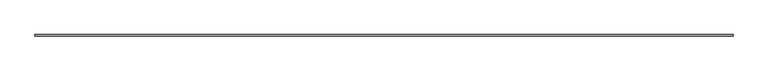
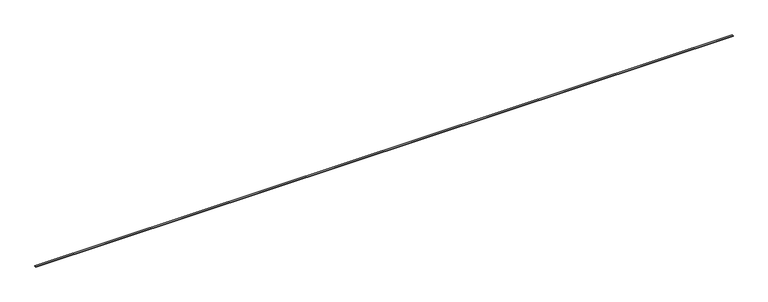
"""IFC4 building model written with IfcOpenShell, lengths in millimetres: proxy geometry, Generic Models 7:Generic Models 1:2:Generic Models 1:2 : Generic Models 7:Generic Models 1:337419:2 : Generic Models 7:Generic Models 1:2:Generic Models 1:2 : Generic Models 7:Generic Models 1:337419:306751."""

from ifc_helpers import new_model, si_unit, frame, origin, place, context, project, spatial, polyline, outline, extrude, source, transform, mapped, element, save


def generic_models_2ad7ca59(model_context):
    return source(origin(), model_context, "Body", "SweptSolid", [
        extrude(outline(polyline([(0.0, -164.8422109), (0.0, 0.0), (76200.0204281, 0.0), (76200.0204281, -164.8422109), (0.0, -164.8422109)])), frame((667506.057152, -567050.5861887, 8571.3891581), z_axis=(0.0, -0.041630544767773385, 0.9991330730900356), x_axis=(-1.0, 0.0, 0.0)), (0.0, 0.0, 1.0), 38.1),
    ])


if __name__ == "__main__":
    model = new_model("IFC4")
    model_context = context("Model", 3, world=origin())
    ifc_project = project(units=[si_unit("LENGTHUNIT", "METRE", prefix="MILLI")], contexts=[model_context])
    site = spatial("IfcSite", under=ifc_project)
    building = spatial("IfcBuilding", under=site)
    placement = place(None, origin())
    generic_models_shape = generic_models_2ad7ca59(model_context)
    element("IfcBuildingElementProxy", 1, Name="Generic Models 7:Generic Models 1:2:Generic Models 1:2 : Generic Models 7:Generic Models 1:337419:2 : Generic Models 7:Generic Models 1:2:Generic Models 1:2 : Generic Models 7:Generic Models 1:337419:306751", ObjectType="Generic Models 7:Generic Models 1:2:Generic Models 1:2 : Generic Models 7:Generic Models 1:337419:2 : Generic Models 7:Generic Models 1:2:Generic Models 1:2 : Generic Models 7:Generic Models 1:337419:306751", at=placement, inside=building, context=model_context, shape_type="MappedRepresentation", body=[
        mapped(generic_models_shape, transform((0.0, 0.0, 0.0), x_axis=(1.0, 0.0, 0.0), y_axis=(0.0, 1.0, 0.0), z_axis=(0.0, 0.0, 1.0))),
    ])
    save(model, "model.ifc")

# Revit data of these elements
# Type "Generic Models 7:Generic Models 1:2:Generic Models 1:2 : Generic Models 7:Generic Models 1:337419:2 : Generic Models 7:Generic Models 1:2:Generic Models 1:2 : Generic Models 7:Generic Models 1:337419:306751"
#   NameOverride = "Generic Models 7:Generic Models 1:2:Generic Models 1:2 : Generic Models 7:Generic Models 1:337419:306751"
#   ObjectTypeOverride = "Generic Models 1:2 : Generic Models 7:Generic Models 1:337419"
#   Reference = "Generic Models 1"
#   Tag = "306751"
# Element 1 (IfcBuildingElementProxy, "Generic Models 7:Generic Models 1:2:Generic Models 1:2 : Generic Models 7:Generic Models 1:337419:2 : Generic Models 7:Generic Models 1:2:Generic Models 1:2 : Generic Models 7:Generic Models 1:337419:306751")
#   Materials on its faces: "FIRE RETARDTANT WOOD BLOCKING - SIZE AS NEC."
# Materials
#   "FIRE RETARDTANT WOOD BLOCKING - SIZE AS NEC.": class "Wood", colour RGB 144 113 62, transparency 0, Description = "Pinus Echinata", Cost = 0
